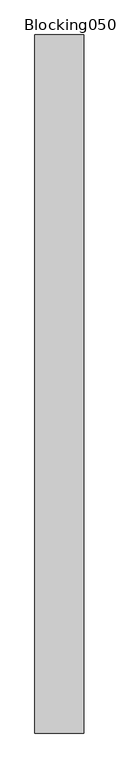
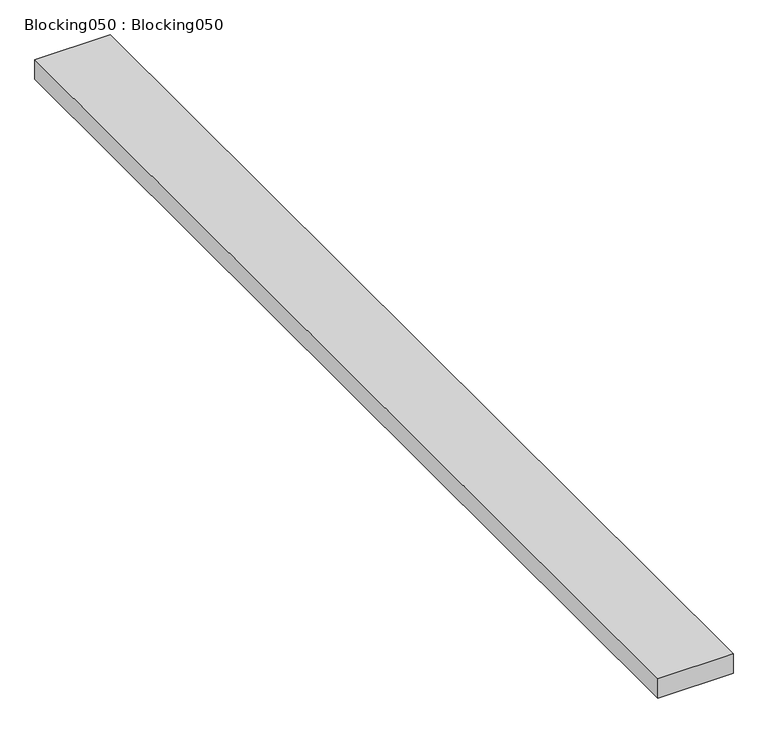
"""IFC4 building model written with IfcOpenShell, lengths in millimetres: proxy geometry, Blocking050 : Blocking050."""

from ifc_helpers import new_model, si_unit, frame, origin, place, context, project, spatial, polyline, outline, extrude, source, transform, mapped, element, save


def blocking050_blocking050_9a0f042f(model_context):
    return source(origin(), model_context, "Body", "SweptSolid", [
        extrude(outline(polyline([(-9501.574441, 7982.1529359), (-9641.274441, 7982.1529359), (-9641.274441, 9982.1529359), (-9501.574441, 9982.1529359), (-9501.574441, 7982.1529359)])), frame((0.0, 0.0, 32568.8960253), z_axis=(0.0, 0.0, 1.0), x_axis=(1.0, 0.0, 0.0)), (0.0, 0.0, 1.0), 38.1),
    ])


if __name__ == "__main__":
    model = new_model("IFC4")
    model_context = context("Model", 3, world=origin())
    ifc_project = project(units=[si_unit("LENGTHUNIT", "METRE", prefix="MILLI")], contexts=[model_context])
    site = spatial("IfcSite", under=ifc_project)
    building = spatial("IfcBuilding", under=site)
    placement = place(None, origin())
    blocking050_blocking050_shape = blocking050_blocking050_9a0f042f(model_context)
    element("IfcBuildingElementProxy", 1, Name="Blocking050 : Blocking050", ObjectType="Blocking050 : Blocking050", at=placement, inside=building, context=model_context, shape_type="MappedRepresentation", body=[
        mapped(blocking050_blocking050_shape, transform((0.0, 0.0, 0.0), x_axis=(1.0, 0.0, 0.0), y_axis=(0.0, 1.0, 0.0), z_axis=(0.0, 0.0, 1.0))),
    ])
    save(model, "model.ifc")

# Revit data of these elements
# Type "Blocking050 : Blocking050"
#   NameOverride = "Blocking050"
# Element 1 (IfcBuildingElementProxy, "Blocking050 : Blocking050")
#   Materials on its faces: "WOOD BLOCKING AS REQUIRED"
# Materials
#   "WOOD BLOCKING AS REQUIRED": class "Unassigned", colour RGB 166 124 85, transparency 0, Cost = 0
